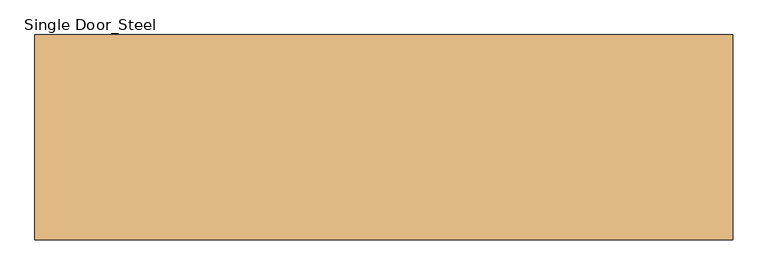
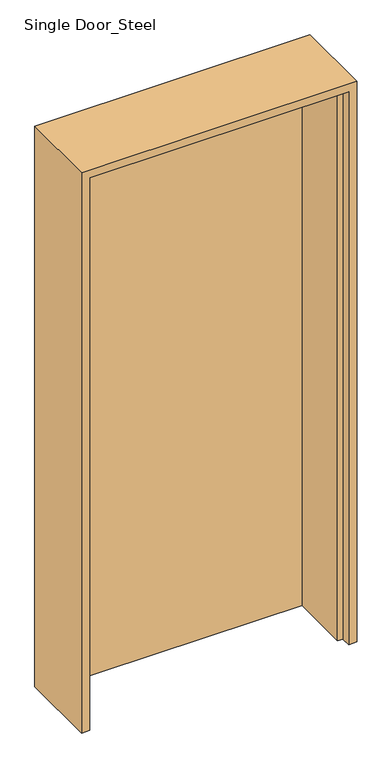
"""IFC4 building model written with IfcOpenShell, lengths in millimetres: door geometry, Single Door_Steel : H_DR_AMB_Single Door_Steel_W1000xH2150."""

import ifcopenshell
import ifcopenshell.guid

model = None  # the IFC model being written
_history = None  # IfcOwnerHistory: only IFC2X3 demands one
_inside = {}  # id of a spatial element -> (the spatial element, [elements in it])
_under = {}  # id of a project, library or spatial element -> (it, [spatial elements below it])
_declared = {}  # id of a project -> (the project, [libraries it declares])
_typed = {}  # id of a type object -> (the type object, [elements of that type])
_made_of = {}  # id of a material, layer set ... -> (it, [elements and type objects made of it])


def new_model(schema):
    """Start an empty IFC model of exactly this schema.

    Asked for "IFC4X3", IfcOpenShell would pick the latest addendum, in which some entities
    have other attributes; the version numbers below select the first issue.
    IFC2X3 requires an IfcOwnerHistory on every rooted entity: one is made here for all.
    """
    global model, _history
    if schema == "IFC4X3":
        model = ifcopenshell.file(schema_version=(4, 3, 0, 0))
    else:
        model = ifcopenshell.file(schema=schema)
    _inside.clear()
    _under.clear()
    _declared.clear()
    _typed.clear()
    _made_of.clear()
    _history = None
    if model.schema == "IFC2X3":
        org = make("IfcOrganization", Name="unknown")
        user = make(
            "IfcPersonAndOrganization",
            ThePerson=make("IfcPerson", FamilyName="unknown"),
            TheOrganization=org,
        )
        app = make(
            "IfcApplication",
            ApplicationDeveloper=org,
            Version="unknown",
            ApplicationFullName="unknown",
            ApplicationIdentifier="unknown",
        )
        _history = make(
            "IfcOwnerHistory",
            OwningUser=user,
            OwningApplication=app,
            ChangeAction="ADDED",
            CreationDate=0,
        )
    return model


def make(cls, **values):
    """One entity of the class cls with the attributes given. An attribute that is None is left unset."""
    return model.create_entity(
        cls, **{name: value for name, value in values.items() if value is not None}
    )


def rooted(cls, **values):
    """An entity with a GlobalId (a new one), such as an element, a storey or a relation."""
    return make(cls, GlobalId=ifcopenshell.guid.new(), OwnerHistory=_history, **values)


def si_unit(unit_type, name, prefix=None):
    """IfcSIUnit, for example si_unit("LENGTHUNIT", "METRE", prefix="MILLI")."""
    return make("IfcSIUnit", UnitType=unit_type, Prefix=prefix, Name=name)


def assignment(units):
    """IfcUnitAssignment: the units of a project."""
    return None if units is None else make("IfcUnitAssignment", Units=units)


def point(xyz):
    """IfcCartesianPoint."""
    return None if xyz is None else make("IfcCartesianPoint", Coordinates=xyz)


def direction(xyz):
    """IfcDirection."""
    return None if xyz is None else make("IfcDirection", DirectionRatios=xyz)


def frame(location, z_axis=None, x_axis=None):
    """IfcAxis2Placement3D, a coordinate frame: its origin and axes. An axis left out is left unset."""
    return make(
        "IfcAxis2Placement3D",
        Location=point(location),
        Axis=direction(z_axis),
        RefDirection=direction(x_axis),
    )


def origin():
    """The frame at (0, 0, 0) with its axes left unset."""
    return frame((0.0, 0.0, 0.0))


def origin_with_axes():
    """The frame at (0, 0, 0) with the z axis (0, 0, 1) and the x axis (1, 0, 0) written out."""
    return frame((0.0, 0.0, 0.0), z_axis=(0.0, 0.0, 1.0), x_axis=(1.0, 0.0, 0.0))


def place(relative_to, where):
    """IfcLocalPlacement: puts the frame where relative to a parent placement (None: the world)."""
    return make(
        "IfcLocalPlacement", PlacementRelTo=relative_to, RelativePlacement=where
    )


def context(
    kind, dimensions, precision=None, world=None, true_north=None, identifier=None
):
    """IfcGeometricRepresentationContext, for example the 3D "Model" context."""
    return make(
        "IfcGeometricRepresentationContext",
        ContextIdentifier=identifier,
        ContextType=kind,
        CoordinateSpaceDimension=dimensions,
        Precision=precision,
        WorldCoordinateSystem=world,
        TrueNorth=true_north,
    )


def project(units=None, contexts=None):
    """IfcProject with its units and contexts."""
    return rooted(
        "IfcProject",
        Name="project",
        RepresentationContexts=contexts,
        UnitsInContext=assignment(units),
    )


def spatial(cls, under=None, at=None, **own):
    """A site, building, storey or space (cls), placed at a placement, below another one or the project."""
    s = rooted(cls, ObjectPlacement=at, **own)
    if under is not None:
        _under.setdefault(under.id(), (under, []))[1].append(s)
    return s


def polyline(points):
    """IfcPolyline through the points."""
    return make("IfcPolyline", Points=[point(p) for p in points])


def outline(outer, holes=None, kind="AREA"):
    """IfcArbitraryClosedProfileDef: a profile drawn as a closed curve; with holes, ...WithVoids."""
    if holes is None:
        return make("IfcArbitraryClosedProfileDef", ProfileType=kind, OuterCurve=outer)
    return make(
        "IfcArbitraryProfileDefWithVoids",
        ProfileType=kind,
        OuterCurve=outer,
        InnerCurves=holes,
    )


def extrude(swept, where, along, depth):
    """IfcExtrudedAreaSolid: the profile swept, set in the frame where, extruded along a direction by depth."""
    return make(
        "IfcExtrudedAreaSolid",
        SweptArea=swept,
        Position=where,
        ExtrudedDirection=direction(along),
        Depth=depth,
    )


def faces_of(points, faces, orient=None, outer=None):
    """IfcFace entities. A face is a list of loops; a loop is a list of indices into points, from 0.

    orient and outer hold one flag for each loop. By default every Orientation is true, the
    first loop of a face is its IfcFaceOuterBound and the others are IfcFaceBound.
    """
    made = []
    for i, loops in enumerate(faces):
        bounds = []
        for j, loop in enumerate(loops):
            is_outer = j == 0 if outer is None else outer[i][j]
            bounds.append(
                make(
                    "IfcFaceOuterBound" if is_outer else "IfcFaceBound",
                    Bound=make("IfcPolyLoop", Polygon=[points[k] for k in loop]),
                    Orientation=True if orient is None else orient[i][j],
                )
            )
        made.append(make("IfcFace", Bounds=bounds))
    return made


def faceted_brep(points, faces, orient=None, outer=None, voids=None):
    """IfcFacetedBrep: a solid bounded by flat faces; with voids (closed shells), ...WithVoids."""
    shared = [point(p) for p in points]
    hull = make("IfcClosedShell", CfsFaces=faces_of(shared, faces, orient, outer))
    if voids is None:
        return make("IfcFacetedBrep", Outer=hull)
    return make(
        "IfcFacetedBrepWithVoids",
        Outer=hull,
        Voids=[
            make(cls, CfsFaces=faces_of(shared, fs, o, b)) for cls, fs, o, b in voids
        ],
    )


def shape(context_of_items, identifier, shape_type, items):
    """IfcShapeRepresentation: the items that make up one representation, for example the "Body"."""
    return make(
        "IfcShapeRepresentation",
        ContextOfItems=context_of_items,
        RepresentationIdentifier=identifier,
        RepresentationType=shape_type,
        Items=items,
    )


def source(mapping_origin, context_of_items, identifier, shape_type, items):
    """IfcRepresentationMap: a shape defined once, which mapped items show again and again."""
    return make(
        "IfcRepresentationMap",
        MappingOrigin=mapping_origin,
        MappedRepresentation=shape(context_of_items, identifier, shape_type, items),
    )


def transform(
    local_origin,
    x_axis=None,
    y_axis=None,
    z_axis=None,
    scale=None,
    scale2=None,
    scale3=None,
    uniform=True,
):
    """IfcCartesianTransformationOperator3D, or its non-uniform kind. x_axis, y_axis, z_axis: its Axis1, 2, 3."""
    if uniform:
        return make(
            "IfcCartesianTransformationOperator3D",
            Axis1=direction(x_axis),
            Axis2=direction(y_axis),
            LocalOrigin=point(local_origin),
            Scale=scale,
            Axis3=direction(z_axis),
        )
    return make(
        "IfcCartesianTransformationOperator3DnonUniform",
        Axis1=direction(x_axis),
        Axis2=direction(y_axis),
        LocalOrigin=point(local_origin),
        Scale=scale,
        Axis3=direction(z_axis),
        Scale2=scale2,
        Scale3=scale3,
    )


def mapped(mapping_source, mapping_target):
    """IfcMappedItem: shows the shape of a source again, moved by a transform."""
    return make(
        "IfcMappedItem", MappingSource=mapping_source, MappingTarget=mapping_target
    )


def made_of(thing, what):
    """Note that an element or type object is made of a material, layer set ...; save() writes the relation."""
    if what is not None:
        _made_of.setdefault(what.id(), (what, []))[1].append(thing)
    return thing


def element(
    cls,
    number,
    at=None,
    inside=None,
    cuts=None,
    type_object=None,
    material=None,
    context=None,
    identifier="Body",
    shape_type=None,
    held_by="IfcProductDefinitionShape",
    body=None,
    shapes=None,
    **own,
):
    """One element of the class cls, such as IfcWall. Its Tag is "e" and its number.

    at: its placement. inside: the storey or other place that contains it. cuts: it is an
    opening in that element (IfcRelVoidsElement). A single representation is given by context,
    identifier, shape_type and body (its items); several are given by shapes. held_by: the class
    of the entity that holds the representations. save() writes the other relations.
    """
    e = rooted(cls, Tag="e%d" % number, ObjectPlacement=at, **own)
    if body is not None:
        shapes = [shape(context, identifier, shape_type, body)]
    if shapes is not None:
        e.Representation = make(held_by, Representations=shapes)
    if inside is not None:
        _inside.setdefault(inside.id(), (inside, []))[1].append(e)
    if cuts is not None:
        rooted(
            "IfcRelVoidsElement", RelatingBuildingElement=cuts, RelatedOpeningElement=e
        )
    if type_object is not None:
        _typed.setdefault(type_object.id(), (type_object, []))[1].append(e)
    return made_of(e, material)


def aggregate(whole, parts):
    """IfcRelAggregates: a whole, such as a stair, and the parts it consists of."""
    return rooted("IfcRelAggregates", RelatingObject=whole, RelatedObjects=parts)


def save(model, path):
    """Write the relations noted so far, then the file.

    IfcRelAggregates (storeys below a building ...), IfcRelContainedInSpatialStructure (elements
    in a storey), IfcRelDefinesByType, IfcRelAssociatesMaterial and IfcRelDeclares: one each for
    every whole, place, type object, material and project.
    """
    for whole, parts in _under.values():
        aggregate(whole, parts)
    for where, things in _inside.values():
        rooted(
            "IfcRelContainedInSpatialStructure",
            RelatedElements=things,
            RelatingStructure=where,
        )
    for kind, things in _typed.values():
        rooted("IfcRelDefinesByType", RelatedObjects=things, RelatingType=kind)
    for what, things in _made_of.values():
        rooted("IfcRelAssociatesMaterial", RelatedObjects=things, RelatingMaterial=what)
    for by, libraries in _declared.values():
        rooted("IfcRelDeclares", RelatingContext=by, RelatedDefinitions=libraries)
    model.write(path)


def single_door_steel_d38beafa(model_context):
    return source(origin(), model_context, "Body", "SolidModel", [
        extrude(outline(polyline([(470.0, 147.0), (470.0, 112.0), (-470.0, 112.0), (-470.0, 147.0), (470.0, 147.0)])), origin_with_axes(), (0.0, 0.0, 1.0), 2120.0),
        faceted_brep([(470.0, 147.0, 0.0), (500.0, 147.0, 0.0), (500.0, -147.0, 0.0), (470.0, -147.0, 0.0), (470.0, -112.0, 0.0), (450.0, -112.0, 0.0), (450.0, 112.0, 0.0), (470.0, 112.0, 0.0), (470.0, 147.0, 2120.0), (-470.0, 147.0, 2120.0), (-470.0, 147.0, 0.0), (-500.0, 147.0, 0.0), (-500.0, 147.0, 2150.0), (500.0, 147.0, 2150.0), (500.0, -147.0, 2150.0), (-500.0, -147.0, 2150.0), (-500.0, -147.0, 0.0), (-470.0, -147.0, 0.0), (-470.0, -147.0, 2120.0), (470.0, -147.0, 2120.0), (470.0, -112.0, 2120.0), (-470.0, -112.0, 2120.0), (-470.0, -112.0, 0.0), (-450.0, -112.0, 0.0), (-450.0, -112.0, 2100.0), (450.0, -112.0, 2100.0), (450.0, 112.0, 2100.0), (-450.0, 112.0, 2100.0), (-450.0, 112.0, 0.0), (-470.0, 112.0, 0.0), (-470.0, 112.0, 2120.0), (470.0, 112.0, 2120.0)], [[[0, 1, 2, 3, 4, 5, 6, 7]], [[1, 0, 8, 9, 10, 11, 12, 13]], [[2, 1, 13, 14]], [[3, 2, 14, 15, 16, 17, 18, 19]], [[4, 3, 19, 20]], [[5, 4, 20, 21, 22, 23, 24, 25]], [[6, 5, 25, 26]], [[7, 6, 26, 27, 28, 29, 30, 31]], [[0, 7, 31, 8]], [[9, 30, 29, 10]], [[10, 29, 28, 23, 22, 17, 16, 11]], [[15, 12, 11, 16]], [[21, 18, 17, 22]], [[27, 24, 23, 28]], [[14, 13, 12, 15]], [[20, 19, 18, 21]], [[26, 25, 24, 27]], [[8, 31, 30, 9]]]),
    ])


if __name__ == "__main__":
    model = new_model("IFC4")
    model_context = context("Model", 3, world=origin())
    ifc_project = project(units=[si_unit("LENGTHUNIT", "METRE", prefix="MILLI")], contexts=[model_context])
    site = spatial("IfcSite", under=ifc_project)
    building = spatial("IfcBuilding", under=site)
    placement = place(None, origin())
    single_door_steel_shape = single_door_steel_d38beafa(model_context)
    element("IfcDoor", 1, ObjectType="Single Door_Steel : H_DR_AMB_Single Door_Steel_W1000xH2150", at=placement, inside=building, context=model_context, shape_type="MappedRepresentation", body=[
        mapped(single_door_steel_shape, transform((0.0, 0.0, 0.0), x_axis=(1.0, 0.0, 0.0), y_axis=(0.0, 1.0, 0.0), z_axis=(0.0, 0.0, 1.0))),
    ])
    save(model, "model.ifc")

# Revit data of these elements
# Type "Single Door_Steel : H_DR_AMB_Single Door_Steel_W1000xH2150"
#   Type Mark = "364"
#   Analytic Construction = "<None>"
#   프레임 투영 외부. = 25.000 mm
#   프레임 투영 내부. = 25.000 mm
#   프레임 폭 = 75.000 mm
#   Height = 2150.000 mm
#   Width = 1000.000 mm
#   Define Thermal Properties by = 1
#   문 패널 = none
#   문 프레임 = none
#   Function = (empty or 0)
#   Wall Closure = (empty or 0)
